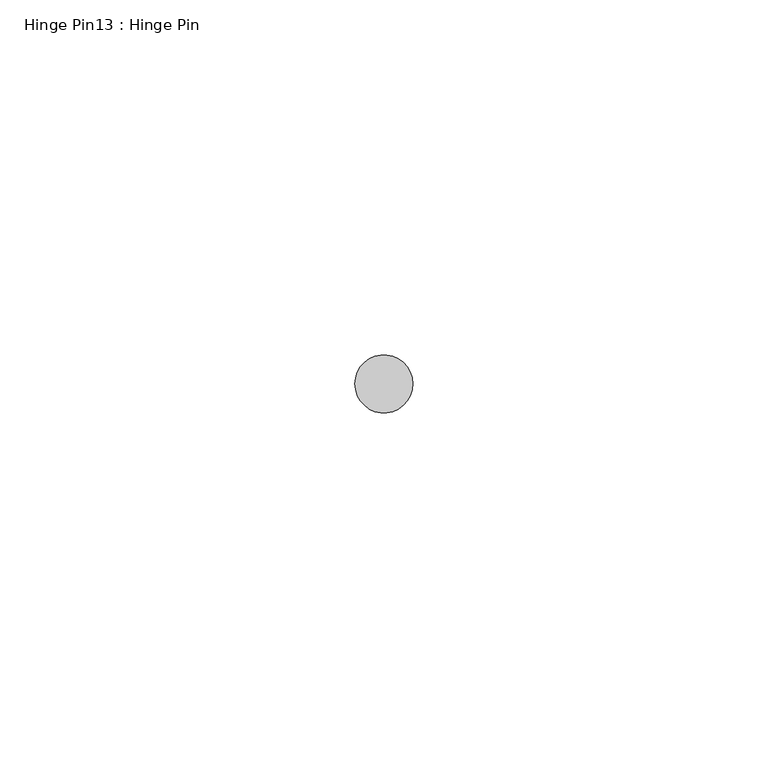
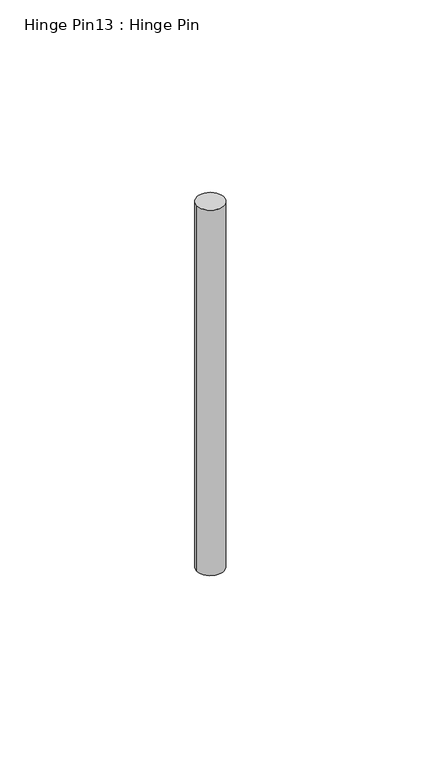
"""IFC4 building model written with IfcOpenShell, lengths in millimetres: proxy geometry, Hinge Pin13 : Hinge Pin."""

from ifc_helpers import new_model, si_unit, point, frame, frame_2d, origin, place, context, project, spatial, circle_curve, trimmed, segment, composite_curve, outline, extrude, source, transform, mapped, element, save


def hinge_pin13_hinge_pin_c6ae77a8(model_context):
    return source(origin(), model_context, "Body", "SweptSolid", [
        extrude(outline(composite_curve([segment(trimmed(circle_curve(frame_2d((587319.1320739, -531776.6049841)), 4.0894), [point((587315.0426739, -531776.6049841))], [point((587323.2214739, -531776.6049841))], False, "CARTESIAN"), True, "CONTINUOUS"), segment(trimmed(circle_curve(frame_2d((587319.1320739, -531776.6049841)), 4.0894), [point((587323.2214739, -531776.6049841))], [point((587315.0426739, -531776.6049841))], False, "CARTESIAN"), True, "CONTINUOUS")], self_intersect=False)), frame((0.0, 0.0, 1941.3140625), z_axis=(0.0, 0.0, 1.0), x_axis=(1.0, 0.0, 0.0)), (0.0, 0.0, 1.0), 117.871875),
    ])


if __name__ == "__main__":
    model = new_model("IFC4")
    model_context = context("Model", 3, world=origin())
    ifc_project = project(units=[si_unit("LENGTHUNIT", "METRE", prefix="MILLI")], contexts=[model_context])
    site = spatial("IfcSite", under=ifc_project)
    building = spatial("IfcBuilding", under=site)
    placement = place(None, origin())
    hinge_pin13_hinge_pin_shape = hinge_pin13_hinge_pin_c6ae77a8(model_context)
    element("IfcBuildingElementProxy", 1, Name="Hinge Pin13 : Hinge Pin", ObjectType="Hinge Pin13 : Hinge Pin", at=placement, inside=building, context=model_context, shape_type="MappedRepresentation", body=[
        mapped(hinge_pin13_hinge_pin_shape, transform((0.0, 0.0, 0.0), x_axis=(1.0, 0.0, 0.0), y_axis=(0.0, 1.0, 0.0), z_axis=(0.0, 0.0, 1.0))),
    ])
    save(model, "model.ifc")

# Revit data of these elements
# Element 1 (IfcBuildingElementProxy, "Hinge Pin13 : Hinge Pin")
#   Materials on its faces: "6\"X6\" WELD-ON STL BUTT HINGE"
# Materials
#   "6\"X6\" WELD-ON STL BUTT HINGE": class "Metal", colour RGB 189 187 185, transparency 0, Description = "Carbon steel", Cost = 0
